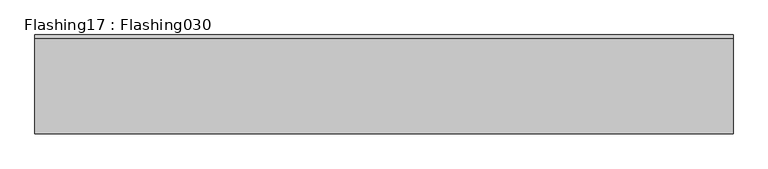
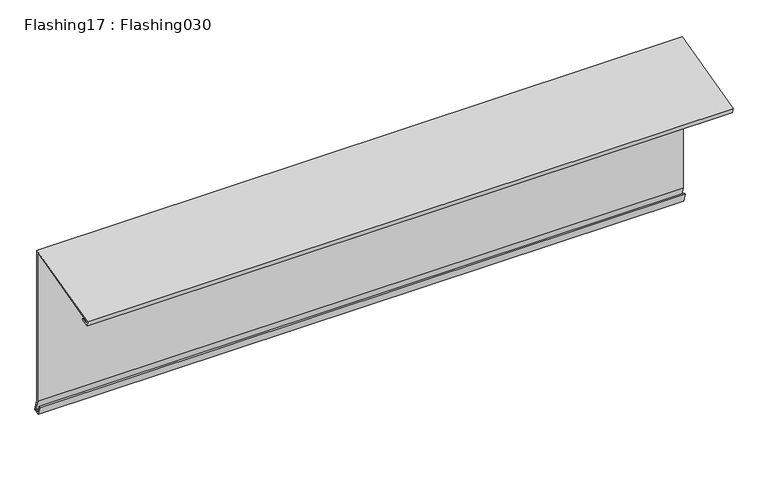
"""IFC4 building model written with IfcOpenShell, lengths in millimetres: proxy geometry, Flashing17 : Flashing030."""

from ifc_helpers import new_model, si_unit, frame, origin, place, context, project, spatial, polyline, outline, extrude, source, transform, mapped, element, save


def flashing17_flashing030_3de79948(model_context):
    return source(origin(), model_context, "Body", "SweptSolid", [
        extrude(outline(polyline([(2022.7017922, 44750.9126137), (2019.2994485, 44765.8813637), (2291.8502297, 44835.5141762), (2291.8502297, 44343.1666992), (2303.0235471, 44306.7687568), (2285.4615579, 44301.3776367), (2276.9400735, 44328.9010742), (2280.7611259, 44330.0841037), (2288.1040277, 44306.3673555), (2298.0315655, 44309.4000801), (2287.8502297, 44342.566566), (2287.8502297, 44830.3637513), (2024.0632268, 44762.9699583), (2025.7058686, 44755.7430887), (2047.4039602, 44760.9280787), (2048.3336282, 44757.0376137), (2022.7017922, 44750.9126137)])), frame((6470.1466437, 0.0, 0.0), z_axis=(1.0, 0.0, 0.0), x_axis=(0.0, 1.0, 0.0)), (0.0, 0.0, 1.0), 1999.85),
    ])


if __name__ == "__main__":
    model = new_model("IFC4")
    model_context = context("Model", 3, world=origin())
    ifc_project = project(units=[si_unit("LENGTHUNIT", "METRE", prefix="MILLI")], contexts=[model_context])
    site = spatial("IfcSite", under=ifc_project)
    building = spatial("IfcBuilding", under=site)
    placement = place(None, origin())
    flashing17_flashing030_shape = flashing17_flashing030_3de79948(model_context)
    element("IfcBuildingElementProxy", 1, Name="Flashing17 : Flashing030", ObjectType="Flashing17 : Flashing030", at=placement, inside=building, context=model_context, shape_type="MappedRepresentation", body=[
        mapped(flashing17_flashing030_shape, transform((0.0, 0.0, 0.0), x_axis=(1.0, 0.0, 0.0), y_axis=(0.0, 1.0, 0.0), z_axis=(0.0, 0.0, 1.0))),
    ])
    save(model, "model.ifc")

# Revit data of these elements
# Type "Flashing17 : Flashing030"
#   NameOverride = "Flashing030"
# Element 1 (IfcBuildingElementProxy, "Flashing17 : Flashing030")
#   Materials on its faces: "BRAKE METAL EAVE TRIM TO MATCH STANDING SEAM COLOR"
# Materials
#   "BRAKE METAL EAVE TRIM TO MATCH STANDING SEAM COLOR": class "Unassigned", colour RGB 128 128 128, transparency 0, Cost = 0
